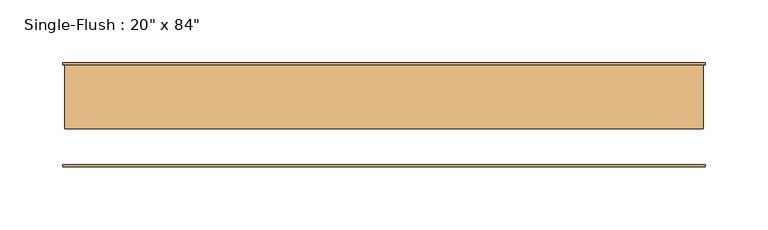
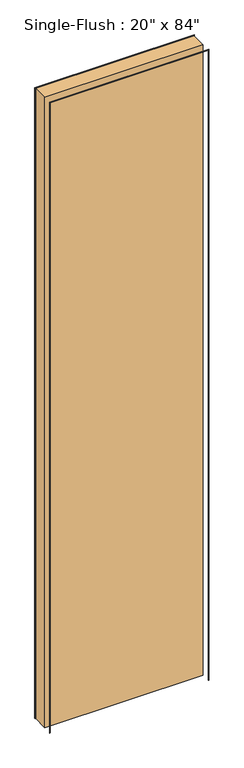
"""IFC4 building model written with IfcOpenShell, lengths in millimetres: door geometry."""

from ifc_helpers import new_model, si_unit, frame, origin, origin_with_axes, place, context, project, spatial, polyline, outline, extrude, source, transform, mapped, element, save


def door_07ed0dde(model_context):
    return source(origin(), model_context, "Body", "SweptSolid", [
        extrude(outline(polyline([(2135.1875, -255.5875), (0.0, -255.5875), (0.0, -254.0), (2133.6, -254.0), (2133.6, 254.0), (0.0, 254.0), (0.0, 255.5875), (2135.1875, 255.5875), (2135.1875, -255.5875)])), frame((0.0, 39.6875, 0.0), z_axis=(0.0, 1.0, 0.0), x_axis=(0.0, 0.0, 1.0)), (0.0, 0.0, 1.0), 1.5875),
        extrude(outline(polyline([(2135.1875, 255.5875), (2135.1875, -255.5875), (0.0, -255.5875), (0.0, -254.0), (2133.6, -254.0), (2133.6, 254.0), (0.0, 254.0), (0.0, 255.5875), (2135.1875, 255.5875)])), frame((0.0, -41.275, 0.0), z_axis=(0.0, 1.0, 0.0), x_axis=(0.0, 0.0, 1.0)), (0.0, 0.0, 1.0), 1.5875),
        extrude(outline(polyline([(254.0, -11.1125), (-254.0, -11.1125), (-254.0, 39.6875), (254.0, 39.6875), (254.0, -11.1125)])), origin_with_axes(), (0.0, 0.0, 1.0), 2133.6),
    ])


if __name__ == "__main__":
    model = new_model("IFC4")
    model_context = context("Model", 3, world=origin())
    ifc_project = project(units=[si_unit("LENGTHUNIT", "METRE", prefix="MILLI")], contexts=[model_context])
    site = spatial("IfcSite", under=ifc_project)
    building = spatial("IfcBuilding", under=site)
    placement = place(None, origin())
    door_shape = door_07ed0dde(model_context)
    element("IfcDoor", 1, ObjectType="Single-Flush : 20\" x 84\"", at=placement, inside=building, context=model_context, shape_type="MappedRepresentation", body=[
        mapped(door_shape, transform((0.0, 0.0, 0.0), x_axis=(1.0, 0.0, 0.0), y_axis=(0.0, 1.0, 0.0), z_axis=(0.0, 0.0, 1.0))),
    ])
    save(model, "model.ifc")

# Revit data of these elements
# Project information
#   Project Issue Date = "Issue Date"
#   Project Status = "Project Status"
#   Client Name = "Owner"
#   Project Address = "Enter address here"
#   Project Name = "Project Name"
#   Project Number = "Project Number"
#   SR Document GUID = "4bc87e05-88e2-428e-9b18-4d898ac90ae1"
# Type "Single-Flush : 20\" x 84\""
#   Type Mark = "42"
#   Assembly Code = "C1020"
#   Thickness = 0' - 2"
#   Height = 7' - 0"
#   Trim Projection Ext = 0' - 0 1/16"
#   Trim Projection Int = 0' - 0 1/16"
#   Trim Width = 0' - 0 1/16"
#   Width = 1' - 8"
#   Door Material = Door - Panel
#   Frame Material = Door - Frame
#   Function = (empty or 0)
#   Wall Closure = (empty or 0)
# Element 1 (IfcDoor, "Single-Flush : 20\" x 84\"")
#   Materials on its faces: "Door - Frame", "Door - Panel"
# Materials
#   "Door - Panel": class "Wood", colour RGB 210 159 95, transparency 0
#   "Door - Frame": class "Miscellaneous", colour RGB 118 70 51, transparency 0
